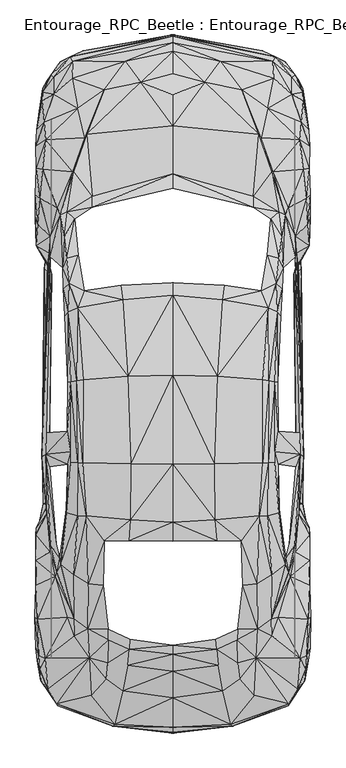
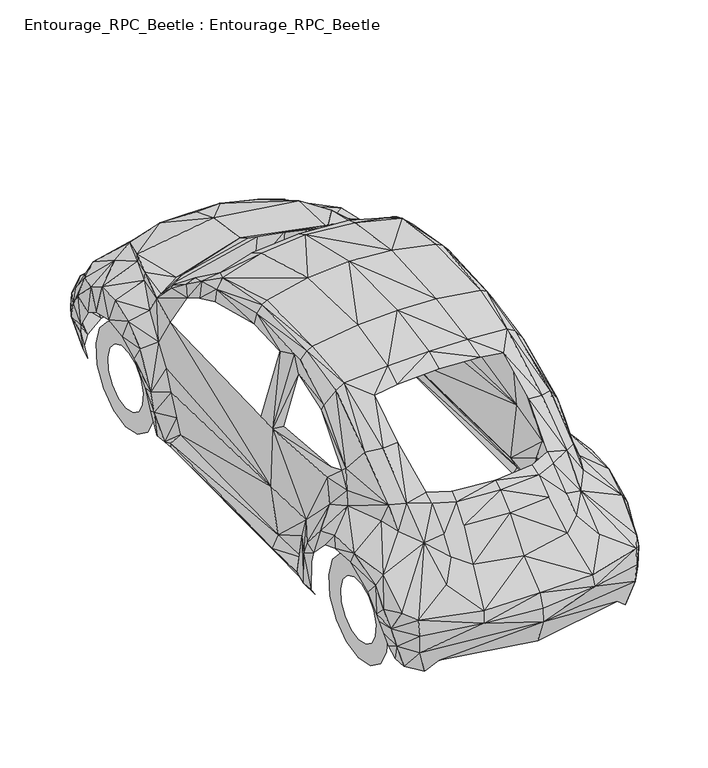
"""IFC4 building model written with IfcOpenShell, lengths in millimetres: proxy geometry, Entourage_RPC_Beetle : Entourage_RPC_Beetle."""

from ifc_helpers import new_model, si_unit, origin, place, context, project, spatial, triangles, source, transform, mapped, element, save


def entourage_rpc_beetle_entourage_rpc_beetle_b6d71803(model_context):
    return source(origin(), model_context, "Body", "Tessellation", [
        triangles([(0.0, -749.071574, 521.742899), (0.0, -720.6335569, 604.033443), (0.0, -697.1470545, 283.3282728), (0.0, -553.0728908, 738.9057701), (0.0, -753.760096, 438.7513078), (0.0, -253.8386484, 1040.4185434), (0.0, -401.3744104, 922.0218458), (0.0, -305.0182643, 1012.9445663), (0.0, 339.5469707, 1396.6602436), (0.0, 448.9171117, 1443.1075539), (0.0, 778.6050184, 1505.0664173), (0.0, 1285.8879353, 1510.4998066), (0.0, 1742.2541199, 1403.2768456), (0.0, 2432.6093651, 967.8556761), (0.0, 3132.1224815, 632.4714237), (0.0, 3003.4724854, 772.0323092), (0.0, 2706.0784286, 929.3833151), (0.0, 3166.3445206, 220.3177475), (0.0, 2885.1195351, 859.3180424), (0.0, 3224.7104347, 396.0724085), (0.0, 3181.1549538, 556.1401817), (0.0, 3216.1220055, 530.6379956), (-338.407687, -715.988855, 523.3642027), (-331.2653541, -702.6243364, 593.8676027), (-244.8997318, -218.1706584, 1034.7659815), (-249.1500901, -276.1420835, 1003.6112698), (-257.9137267, -368.4231514, 912.4695219), (-249.2377301, 343.0524253, 1381.9373051), (-285.431542, -511.8838351, 760.9462852), (-240.2988317, 460.3974792, 1427.552108), (-236.6180971, 781.4093531, 1494.4185207), (-652.9344915, -590.6250681, 370.7455024), (-540.4532759, -593.7361791, 283.6349946), (-181.3633847, 2956.2803078, 806.8677555), (-253.3566466, 1279.4466133, 1497.179108), (-380.1225826, -444.6667534, 798.8051662), (-371.1837024, -353.5687892, 889.7717068), (-368.2478714, -222.3771967, 1004.1371098), (-368.6422514, -160.8126769, 1037.3951088), (-390.4198829, 343.0962453, 1359.9406826), (-282.758631, 1714.4296555, 1400.2533382), (-397.6060358, 87.5486986, 1216.1732225), (-463.4209502, -538.1309249, 705.2972111), (-271.6726434, 3074.4140854, 663.1441154), (-476.0843851, -323.2904411, 850.4230185), (-464.0343939, 3087.9975586, 214.4022838), (-482.5694544, 95.8303334, 1204.2108713), (-485.3738254, -159.4104914, 1005.7583771), (-569.1103566, 3073.5815781, 547.1136251), (-493.874542, 483.577278, 1392.2346416), (-583.6579788, 3101.4935371, 522.400199), (-510.6130915, 3134.4011215, 369.6500387), (-392.1287902, 2913.6012268, 783.2935404), (-656.7905062, -598.249421, 480.4223834), (-660.6903408, -585.2354261, 576.6470695), (-562.669071, -200.2052034, 880.3069502), (-560.43436, -101.5266881, 987.8367239), (-512.8040188, 786.711355, 1449.4173431), (-542.1621832, 485.1109417, 1360.7731899), (-564.3779783, 148.6750366, 1173.0999796), (-608.8972449, -561.6174273, 218.6088402), (-511.6209151, 1259.3779255, 1457.1731197), (-542.7756269, 785.2215477, 1431.62715), (-459.1705556, 2305.6242382, 949.6711029), (-601.448172, -92.8068806, 893.8030014), (-504.0842022, 1766.485635, 1321.8626289), (-546.4125415, 1253.8568962, 1442.4940739), (-603.419963, 501.4989312, 1279.4466133), (-580.5469042, 789.4281223, 1379.6588104), (-607.6265376, 520.2092717, 1235.979063), (-601.6672357, 965.9276688, 1337.9439148), (-712.9654203, -503.4269022, 590.8879881), (-543.0385468, 1671.1811325, 1362.0876446), (-490.9387473, 2659.6751564, 894.1096687), (-600.0459683, 778.6050184, 1308.1913704), (-598.468521, 1244.567347, 1344.6919041), (-640.008173, 208.2677382, 1063.2039986), (-680.8904886, -470.5194632, 218.8279221), (-538.8320086, 1968.0492039, 1181.3815962), (-581.3794478, 1249.0807343, 1402.7071129), (-644.9596149, 243.4537263, 1028.9820322), (-502.6819985, 2637.5907486, 866.5918716), (-661.1722881, 162.3463042, 955.8933249), (-690.7057325, -396.8611321, 226.9780968), (-559.5141764, 2176.4921494, 1011.849139), (-670.6370447, 140.9630437, 873.2960409), (-662.9250154, 324.5173285, 1010.1402317), (-615.5138105, 1624.5585423, 1262.9710201), (-595.0507064, 1647.2125374, 1322.1692963), (-589.8363444, 1810.8295853, 1270.2885967), (-729.3095535, -482.3065707, 373.4622334), (-752.0950087, -454.7449536, 476.8731088), (-694.5179272, 315.5346282, 958.4347395), (-727.0748789, -327.5407994, 736.0575428), (-623.3572271, 1778.4479862, 1193.6068674), (-565.0352783, 2447.3761963, 934.772957), (-732.2892408, -394.1444012, 324.3420848), (-571.3888876, 2445.9300636, 884.7764448), (-699.1188818, 280.0419, 808.1822828), (-604.6907066, 1951.091518, 1171.2596123), (-587.8206971, 3015.1281693, 200.2490234), (-691.4068525, 574.6314222, 283.8102746), (-750.7366613, -381.2618663, 397.2555121), (-627.9581818, 1897.5456585, 1125.469602), (-602.8941593, 2217.067725, 949.8025629), (-619.8517725, 2074.2206303, 1075.9989298), (-710.949773, 550.0056361, 448.9171117), (-765.2404999, -360.5796985, 467.8465522), (-699.9952091, 763.1372126, 1016.187101), (-763.8382599, -313.4313409, 671.3819847), (-758.3609779, -391.2086065, 565.0352783), (-717.9606823, 496.6350929, 583.9647188), (-723.2188643, 461.5367629, 181.1004829), (-718.1359623, 554.8256181, 180.0050374), (-771.9884892, -342.0446016, 511.3579951), (-574.3247186, 2977.4883156, 683.0814159), (-731.2813808, 376.1351443, 185.3070212), (-541.5487395, 2807.2984131, 783.4688204), (-640.183453, 2199.9349045, 944.8949409), (-739.4315374, 551.9336434, 222.5524767), (-782.1104731, -268.9559124, 609.6421486), (-772.8209965, -106.1275973, 756.4330433), (-722.2110043, 958.3909195, 967.6803961), (-703.8074038, 810.6798775, 292.5300731), (-725.3221516, 835.6124399, 965.0075214), (-758.2734106, 370.7893224, 225.6197495), (-785.8788477, -90.0025187, 695.9639145), (-780.1824657, 80.9759712, 676.0266867), (-779.9195457, 89.5643369, 755.1622633), (-760.9024652, 444.4038334, 223.2973804), (-778.6050184, 192.2302905, 631.3321764), (-659.0690735, 2238.6701855, 850.3353785), (-771.4626492, 345.7253363, 426.4822165), (-774.7051838, 315.3593482, 502.0247349), (-781.7160931, 232.4115588, 696.3582945), (-719.7134096, 810.6360575, 185.964303), (-690.3552452, 1860.1249775, 294.1075386), (-697.1470545, 1960.2056419, 957.0763922), (-780.2701057, 377.6249516, 532.7412829), (-778.6488384, 417.2804163, 440.0220151), (-746.0043194, 820.1446341, 614.0678232), (-678.173794, 2886.7845497, 671.0752447), (-698.0233818, 2078.8215122, 757.3970106), (-640.051993, 3071.2590454, 391.9535102), (-713.4911877, 1919.5424263, 537.0792812), (-718.6617296, 1911.1731697, 193.1066541), (-705.6477711, 1983.2978371, 648.7279896), (-731.2813808, 1892.3751892, 233.5070043), (-674.4492393, 2909.8331429, 198.8030179), (-727.3815462, 2040.3052586, 190.0832013), (-722.1233643, 1974.7095531, 190.0832013), (-678.6557413, 2984.5867195, 540.8914395), (-700.0828491, 2817.5957497, 206.339749), (-696.8403145, 2993.6132034, 517.7554607), (-724.1390116, 2626.4609047, 788.1135223), (-699.5570091, 1883.7430126, 390.6389465), (-765.4157072, 2043.5477932, 362.8144094), (-742.2797647, 2459.3385475, 809.2338902), (-716.646155, 2967.1470863, 449.8372953), (-766.9494072, 2002.4902702, 376.836228), (-732.0701408, 2726.2786491, 728.1264862), (-771.6817492, 2086.0077015, 482.5694544), (-759.6317579, 2292.9609123, 780.6206657), (-769.5346418, 2144.7677776, 699.5131891), (-778.0791784, 2024.2239727, 495.1452856), (-742.9808121, 2848.7944267, 602.2807157), (-782.6363131, 2187.1400459, 616.8721579), (-740.0450174, 2920.3932541, 427.6653202), (-741.6224648, 2898.4841263, 520.1654517), (-750.9119413, 2806.3345184, 398.3509395), (-782.7677004, 2314.7385075, 681.1972286), (-778.6050184, 2464.4652695, 693.9921598), (-760.4204453, 2788.5004326, 455.5336773), (-774.7051838, 2684.6515388, 603.0694393), (-780.8835857, 2591.1871857, 666.7810301), (-743.1122721, 809.6720901, 220.5368294), (0.0, 2350.6693085, 1011.849139), (-459.1705556, 2241.4745201, 1007.2920044), (0.0, 1813.2396126, 1369.1424465), (-294.1513586, 1797.0267941, 1360.0720699), (-580.6345442, 850.2915585, 1382.7260651), (338.407687, -715.988855, 523.3642027), (331.2653541, -702.6243364, 593.8676027), (244.8997318, -218.1706584, 1034.7659815), (249.1500901, -276.1420835, 1003.6112698), (257.9137267, -368.4231514, 912.4695219), (249.2377301, 343.0524253, 1381.9373051), (285.431542, -511.8838351, 760.9462852), (240.2988317, 460.3974792, 1427.552108), (236.6180971, 781.4093531, 1494.4185207), (652.9344915, -590.6250681, 370.7455024), (540.4532759, -593.7361791, 283.6349946), (181.3633847, 2956.2803078, 806.8677555), (253.3566466, 1279.4466133, 1497.179108), (380.1225826, -444.6667534, 798.8051662), (371.1837024, -353.5687892, 889.7717068), (368.2478714, -222.3771967, 1004.1371098), (368.6422514, -160.8126769, 1037.3951088), (390.4198829, 343.0962453, 1359.9406826), (282.758631, 1714.4296555, 1400.2533382), (397.6060358, 87.5486986, 1216.1732225), (463.4209502, -538.1309249, 705.2972111), (271.6726434, 3074.4140854, 663.1441154), (476.0843851, -323.2904411, 850.4230185), (464.0343939, 3087.9975586, 214.4022838), (482.5694544, 95.8303334, 1204.2108713), (485.3738254, -159.4104914, 1005.7583771), (569.1103566, 3073.5815781, 547.1136251), (493.874542, 483.577278, 1392.2346416), (583.6579788, 3101.4935371, 522.400199), (510.6130915, 3134.4011215, 369.6500387), (392.1287902, 2913.6012268, 783.2935404), (656.7905062, -598.249421, 480.4223834), (660.6903408, -585.2354261, 576.6470695), (562.669071, -200.2052034, 880.3069502), (560.43436, -101.5266881, 987.8367239), (512.8040188, 786.711355, 1449.4173431), (542.1621832, 485.1109417, 1360.7731899), (564.3779783, 148.6750366, 1173.0999796), (608.8972449, -561.6174273, 218.6088402), (511.6209151, 1259.3779255, 1457.1731197), (542.7756269, 785.2215477, 1431.62715), (459.1705556, 2305.6242382, 949.6711029), (601.448172, -92.8068806, 893.8030014), (504.0842022, 1766.485635, 1321.8626289), (546.4125415, 1253.8568962, 1442.4940739), (603.419963, 501.4989312, 1279.4466133), (580.5469042, 789.4281223, 1379.6588104), (607.6265376, 520.2092717, 1235.979063), (601.6672357, 965.9276688, 1337.9439148), (712.9654203, -503.4269022, 590.8879881), (543.0385468, 1671.1811325, 1362.0876446), (490.9387473, 2659.6751564, 894.1096687), (600.0459683, 778.6050184, 1308.1913704), (598.468521, 1244.567347, 1344.6919041), (640.008173, 208.2677382, 1063.2039986), (680.9343086, -470.5194632, 218.8279221), (538.8320086, 1968.0492039, 1181.3815962), (581.3794478, 1249.0807343, 1402.7071129), (644.9596149, 243.4537263, 1028.9820322), (502.6819985, 2637.5907486, 866.5918716), (661.1722881, 162.3463042, 955.8933249), (690.7057325, -396.8611321, 226.9780968), (559.5141764, 2176.4921494, 1011.849139), (670.6370447, 140.9630437, 873.2960409), (662.9250154, 324.5173285, 1010.1402317), (615.5138105, 1624.5585423, 1262.9710201), (595.0507064, 1647.2125374, 1322.1692963), (589.8363444, 1810.8295853, 1270.2885967), (729.3095535, -482.3065707, 373.4622334), (752.0950087, -454.7449536, 476.8731088), (694.5179272, 315.5346282, 958.4347395), (727.0748789, -327.5407994, 736.0575428), (623.3572271, 1778.4479862, 1193.6068674), (565.0352783, 2447.3761963, 934.772957), (732.2892408, -394.1444012, 324.3420848), (571.3888876, 2445.9300636, 884.7764448), (699.1188818, 280.0419, 808.1822828), (604.6907066, 1951.091518, 1171.2596123), (587.8206971, 3015.1281693, 200.2490234), (691.4068525, 574.6314222, 283.8102746), (750.7366613, -381.2618663, 397.2555121), (627.9581818, 1897.5456585, 1125.469602), (602.8941593, 2217.067725, 949.8025629), (619.8517725, 2074.2206303, 1075.9989298), (710.949773, 550.0056361, 448.9171117), (765.2404999, -360.5796985, 467.8465522), (699.9952091, 763.1372126, 1016.187101), (763.8382599, -313.4313409, 671.3819847), (758.3609779, -391.2086065, 565.0352783), (717.9606823, 496.6350929, 583.9647188), (723.2188643, 461.5367629, 181.1004829), (718.1359623, 554.8256181, 180.0050374), (771.9884892, -342.0446016, 511.3579951), (574.3247186, 2977.4883156, 683.0814159), (731.2813808, 376.1351443, 185.3070212), (541.5487395, 2807.2984131, 783.4688204), (640.183453, 2199.9349045, 944.8949409), (739.4315374, 551.9336434, 222.5524767), (782.1104731, -268.9559124, 609.6421486), (772.8209965, -106.1275973, 756.4330433), (722.2548243, 958.3909195, 967.6803961), (703.8074038, 810.6798775, 292.5300731), (725.3221516, 835.6124399, 965.0075214), (758.2734106, 370.7893224, 225.6197495), (785.8788477, -90.0025187, 695.9639145), (780.1824657, 80.9759712, 676.0266867), (779.9633657, 89.5643369, 755.1622633), (760.9024652, 444.4038334, 223.2973804), (778.6050184, 192.2302905, 631.3321764), (659.0690735, 2238.6701855, 850.3353785), (771.4626492, 345.7253363, 426.4822165), (774.7051838, 315.3593482, 502.0247349), (781.7160931, 232.4115588, 696.3582945), (719.7134096, 810.6360575, 185.964303), (690.3552452, 1860.1249775, 294.1075386), (697.1470545, 1960.2056419, 957.0763922), (780.2701057, 377.6249516, 532.7412829), (778.6488384, 417.2804163, 440.0220151), (746.0043194, 820.1446341, 614.0678232), (678.173794, 2886.7845497, 671.0752447), (698.0233818, 2078.8215122, 757.3970106), (640.051993, 3071.2590454, 391.9535102), (713.4911877, 1919.5424263, 537.0792812), (718.6617296, 1911.1731697, 193.1066541), (705.6477711, 1983.2978371, 648.7279896), (731.2813808, 1892.3751892, 233.5070043), (674.4492393, 2909.8331429, 198.8030179), (727.3815462, 2040.3052586, 190.0832013), (722.1233643, 1974.7095531, 190.0832013), (678.6557413, 2984.5867195, 540.8914395), (700.0828491, 2817.5957497, 206.339749), (696.8403145, 2993.6132034, 517.7554607), (724.1390116, 2626.4609047, 788.1135223), (699.5570091, 1883.7430126, 390.6389465), (765.4157072, 2043.5477932, 362.8144094), (742.2797647, 2459.3385475, 809.2338902), (716.646155, 2967.1470863, 449.8372953), (766.9494072, 2002.4902702, 376.836228), (732.0701408, 2726.2786491, 728.1264862), (771.7255692, 2086.0077015, 482.5694544), (759.6317579, 2292.9609123, 780.6206657), (769.5346418, 2144.7677776, 699.5131891), (778.0791784, 2024.2239727, 495.1452856), (742.9808121, 2848.7944267, 602.2807157), (782.6363131, 2187.1400459, 616.8721579), (740.0450174, 2920.3932541, 427.6653202), (741.6224648, 2898.4841263, 520.1654517), (750.9119413, 2806.3345184, 398.3509395), (782.7677004, 2314.7385075, 681.1972286), (778.6050184, 2464.4652695, 693.9921598), (760.4204453, 2788.5004326, 455.5336773), (774.7051838, 2684.6515388, 603.0694393), (780.8835857, 2591.1871857, 666.7810301), (743.1122721, 809.6720901, 220.5368294), (459.1705556, 2241.4745201, 1007.2920044), (294.1513586, 1797.0267941, 1360.0720699), (580.6345442, 850.2915585, 1382.7260651), (-693.6415998, 2431.9082451, 0.0015117), (-693.6415998, 2431.9082451, 117.9161946), (-693.6415998, 2558.8496246, 26.9935036), (-693.6415998, 2509.4663017, 134.3918332), (-693.6415998, 2663.794091, 103.2371124), (-693.6415998, 2573.6600578, 181.0143508), (-693.6415998, 2728.6886765, 215.6307153), (-693.6415998, 2613.3154861, 249.7212399), (-693.6415998, 2742.2724403, 344.6752187), (-693.6415998, 2621.5972481, 328.5939328), (-693.6415998, 2702.1786667, 468.1109982), (-693.6415998, 2597.102813, 404.0050275), (-693.6415998, 2615.3310608, 564.5109644), (-693.6415998, 2544.0389008, 462.9404563), (-693.6415998, 2496.8028305, 617.3118113), (-693.6415998, 2471.5636734, 495.2344517), (-693.6415998, 2367.0135143, 617.3118113), (-693.6415998, 2392.2528168, 495.2344517), (-693.6415998, 2248.4854294, 564.5109644), (-693.6415998, 2319.7775894, 462.9404563), (-693.6415998, 2161.6378235, 468.1109982), (-693.6415998, 2266.7138226, 404.0050275), (-693.6415998, 2121.5441952, 344.6752187), (-693.6415998, 2242.2193874, 328.5939328), (-693.6415998, 2135.1278137, 215.6307153), (-693.6415998, 2250.501004, 249.7212399), (-693.6415998, 2200.0225445, 103.2371124), (-693.6415998, 2290.1564323, 181.0143508), (-693.6415998, 2304.9670109, 26.9935036), (-693.6415998, 2354.3500431, 134.3918332), (693.6415998, 2431.9082451, 0.0015117), (693.6415998, 2431.9082451, 117.9161946), (693.6415998, 2304.9670109, 26.9935036), (693.6415998, 2354.3500431, 134.3918332), (693.6415998, 2200.0225445, 103.2371124), (693.6415998, 2290.1564323, 181.0143508), (693.6415998, 2135.1278137, 215.6307153), (693.6415998, 2250.501004, 249.7212399), (693.6415998, 2121.5441952, 344.6752187), (693.6415998, 2242.2193874, 328.5939328), (693.6415998, 2161.6378235, 468.1109982), (693.6415998, 2266.7138226, 404.0050275), (693.6415998, 2248.4854294, 564.5109644), (693.6415998, 2319.7775894, 462.9404563), (693.6415998, 2367.0135143, 617.3118113), (693.6415998, 2392.2528168, 495.2344517), (693.6415998, 2496.8028305, 617.3118113), (693.6415998, 2471.5636734, 495.2344517), (693.6415998, 2615.3310608, 564.5109644), (693.6415998, 2544.0389008, 462.9404563), (693.6415998, 2702.1786667, 468.1109982), (693.6415998, 2597.102813, 404.0050275), (693.6415998, 2742.2724403, 344.6752187), (693.6415998, 2621.5972481, 328.5939328), (693.6415998, 2728.6886765, 215.6307153), (693.6415998, 2613.3154861, 249.7212399), (693.6415998, 2663.794091, 103.2371124), (693.6415998, 2573.6600578, 181.0143508), (693.6415998, 2558.8496246, 26.9935036), (693.6415998, 2509.4663017, 134.3918332), (-693.6415998, -13.5836322, 0.0015117), (-693.6415998, -13.5836322, 117.9161946), (-693.6415998, 113.3575975, 26.9935036), (-693.6415998, 63.9745244, 134.3918332), (-693.6415998, 218.3021002, 103.2371124), (-693.6415998, 128.1681397, 181.0143508), (-693.6415998, 283.1968128, 215.6307153), (-693.6415998, 167.8235862, 249.7212399), (-693.6415998, 296.7804495, 344.6752187), (-693.6415998, 176.1052209, 328.5939328), (-693.6415998, 256.6868212, 468.1109982), (-693.6415998, 151.6108585, 404.0050275), (-693.6415998, 169.8392153, 564.5109644), (-693.6415998, 98.5470553, 462.9404563), (-693.6415998, 51.3110713, 617.3118113), (-693.6415998, 26.0718098, 495.2344517), (-693.6415998, -78.4783402, 617.3118113), (-693.6415998, -53.2390741, 495.2344517), (-693.6415998, -197.0064706, 564.5109644), (-693.6415998, -125.7143196, 462.9404563), (-693.6415998, -283.8540765, 468.1109982), (-693.6415998, -178.7781137, 404.0050275), (-693.6415998, -323.9477048, 344.6752187), (-693.6415998, -203.2724762, 328.5939328), (-693.6415998, -310.3640862, 215.6307153), (-693.6415998, -194.9908414, 249.7212399), (-693.6415998, -245.4693737, 103.2371124), (-693.6415998, -155.335395, 181.0143508), (-693.6415998, -140.5248618, 26.9935036), (-693.6415998, -91.1417842, 134.3918332), (693.6415998, -13.5836322, 0.0015117), (693.6415998, -13.5836322, 117.9161946), (693.6415998, -140.5248618, 26.9935036), (693.6415998, -91.1417842, 134.3918332), (693.6415998, -245.4693737, 103.2371124), (693.6415998, -155.335395, 181.0143508), (693.6415998, -310.3640862, 215.6307153), (693.6415998, -194.9908414, 249.7212399), (693.6415998, -323.9477048, 344.6752187), (693.6415998, -203.2724762, 328.5939328), (693.6415998, -283.8540765, 468.1109982), (693.6415998, -178.7781137, 404.0050275), (693.6415998, -197.0064706, 564.5109644), (693.6415998, -125.7143196, 462.9404563), (693.6415998, -78.4783402, 617.3118113), (693.6415998, -53.2390741, 495.2344517), (693.6415998, 51.3110713, 617.3118113), (693.6415998, 26.0718098, 495.2344517), (693.6415998, 169.8392153, 564.5109644), (693.6415998, 98.5470553, 462.9404563), (693.6415998, 256.6868212, 468.1109982), (693.6415998, 151.6108585, 404.0050275), (693.6415998, 296.7804495, 344.6752187), (693.6415998, 176.1052209, 328.5939328), (693.6415998, 283.1968128, 215.6307153), (693.6415998, 167.8235862, 249.7212399), (693.6415998, 218.3021002, 103.2371124), (693.6415998, 128.1681397, 181.0143508), (693.6415998, 113.3575975, 26.9935036), (693.6415998, 63.9745244, 134.3918332)], [[67, 58, 62], [67, 63, 58], [53, 82, 74], [34, 17, 19], [118, 82, 53], [155, 98, 82], [155, 158, 98], [34, 74, 17], [172, 155, 175], [172, 158, 155], [159, 168, 169], [166, 142, 169], [175, 161, 174], [175, 155, 161], [142, 152, 169], [154, 169, 152], [160, 145, 165], [160, 156, 145], [162, 160, 165], [162, 157, 160], [34, 53, 74], [74, 96, 64], [82, 96, 74], [82, 98, 96], [36, 29, 27], [29, 43, 24], [23, 55, 54], [23, 24, 55], [23, 2, 24], [23, 1, 2], [5, 1, 23], [134, 140, 133], [134, 139, 140], [117, 130, 113], [117, 126, 130], [113, 120, 114], [113, 130, 120], [140, 112, 107], [140, 139, 112], [92, 108, 103], [91, 103, 97], [91, 92, 103], [61, 33, 32], [84, 78, 91], [84, 91, 97], [38, 26, 25], [77, 81, 83], [63, 50, 58], [63, 59, 50], [68, 63, 69], [68, 59, 63], [181, 75, 69], [74, 64, 17], [64, 14, 17], [64, 178, 14], [178, 177, 14], [34, 19, 16], [53, 34, 44], [21, 44, 15], [21, 49, 44], [44, 34, 15], [34, 16, 15], [22, 49, 21], [22, 51, 49], [20, 51, 22], [20, 52, 51], [18, 52, 20], [18, 46, 52], [51, 152, 49], [51, 154, 152], [101, 144, 46], [144, 52, 46], [101, 159, 144], [159, 169, 154], [101, 168, 159], [101, 149, 168], [149, 170, 168], [149, 153, 170], [168, 173, 169], [168, 170, 173], [49, 142, 116], [49, 152, 142], [49, 116, 44], [116, 142, 118], [161, 155, 118], [155, 82, 118], [142, 161, 118], [158, 132, 98], [158, 163, 132], [172, 163, 158], [172, 171, 163], [98, 119, 96], [98, 132, 119], [171, 164, 163], [171, 167, 164], [163, 143, 132], [163, 164, 143], [96, 105, 64], [96, 119, 105], [105, 178, 64], [105, 85, 178], [167, 165, 164], [167, 162, 165], [165, 143, 164], [165, 147, 143], [150, 160, 157], [150, 151, 160], [151, 156, 160], [151, 148, 137], [13, 35, 12], [13, 41, 35], [12, 31, 11], [12, 35, 31], [35, 58, 31], [35, 62, 58], [11, 30, 10], [11, 31, 30], [31, 50, 30], [31, 58, 50], [10, 28, 9], [10, 30, 28], [30, 40, 28], [30, 50, 40], [125, 75, 181], [125, 109, 75], [125, 87, 109], [125, 93, 87], [123, 141, 125], [137, 141, 156], [137, 124, 141], [148, 124, 137], [148, 176, 124], [146, 176, 148], [146, 136, 176], [141, 112, 125], [112, 93, 125], [112, 99, 93], [124, 112, 141], [124, 107, 112], [124, 102, 107], [176, 102, 124], [176, 120, 102], [136, 120, 176], [136, 114, 120], [47, 40, 50], [47, 42, 40], [48, 42, 47], [48, 39, 42], [57, 47, 60], [57, 48, 47], [60, 50, 59], [60, 47, 50], [59, 77, 60], [59, 68, 77], [77, 57, 60], [77, 83, 57], [70, 77, 68], [70, 81, 77], [75, 68, 69], [75, 70, 68], [26, 6, 25], [26, 8, 6], [27, 8, 26], [27, 7, 8], [29, 7, 27], [29, 4, 7], [24, 4, 29], [24, 2, 4], [32, 5, 23], [33, 5, 32], [33, 3, 5], [32, 23, 54], [55, 45, 72], [55, 24, 43], [99, 83, 93], [99, 86, 83], [135, 86, 99], [135, 129, 86], [131, 129, 135], [131, 128, 129], [93, 81, 87], [93, 83, 81], [128, 122, 129], [128, 127, 122], [122, 86, 129], [122, 65, 86], [86, 57, 83], [86, 65, 57], [127, 110, 122], [127, 121, 110], [110, 94, 122], [122, 94, 65], [94, 56, 65], [56, 57, 65], [56, 48, 57], [56, 45, 48], [94, 45, 56], [115, 110, 121], [115, 111, 110], [111, 94, 110], [111, 72, 94], [108, 92, 115], [92, 111, 115], [78, 32, 91], [78, 61, 32], [45, 38, 48], [45, 37, 38], [37, 26, 38], [37, 27, 26], [36, 27, 37], [134, 135, 139], [134, 131, 135], [139, 99, 112], [139, 135, 99], [126, 140, 130], [126, 133, 140], [130, 107, 120], [130, 140, 107], [120, 107, 102], [45, 36, 37], [92, 55, 72], [92, 54, 55], [91, 54, 92], [91, 32, 54], [92, 72, 111], [72, 45, 94], [43, 45, 55], [43, 36, 45], [43, 29, 36], [79, 90, 66], [79, 100, 90], [90, 73, 66], [85, 100, 79], [85, 106, 100], [85, 105, 106], [105, 119, 106], [95, 88, 89], [90, 89, 73], [89, 67, 73], [73, 67, 62], [89, 76, 80], [89, 80, 67], [88, 76, 89], [73, 35, 41], [73, 62, 35], [69, 63, 181], [80, 63, 67], [76, 71, 80], [146, 148, 151], [141, 147, 145], [151, 137, 156], [173, 166, 169], [173, 174, 166], [166, 174, 161], [166, 161, 142], [52, 144, 51], [144, 154, 51], [144, 159, 154], [116, 53, 44], [116, 118, 53], [119, 143, 138], [143, 119, 132], [143, 147, 138], [138, 104, 119], [119, 104, 106], [104, 100, 106], [104, 90, 100], [104, 95, 90], [95, 89, 90], [25, 39, 38], [38, 39, 48], [141, 138, 147], [156, 141, 145], [165, 145, 147], [41, 179, 180], [41, 13, 179], [66, 41, 180], [66, 73, 41], [123, 125, 71], [125, 181, 71], [71, 181, 80], [181, 63, 80], [138, 141, 123], [226, 221, 217], [226, 217, 222], [212, 233, 241], [193, 19, 17], [277, 212, 241], [314, 241, 257], [314, 257, 317], [193, 17, 233], [331, 334, 314], [331, 314, 317], [318, 328, 327], [325, 328, 301], [334, 333, 320], [334, 320, 314], [301, 328, 311], [313, 311, 328], [319, 324, 304], [319, 304, 315], [321, 324, 319], [321, 319, 316], [193, 233, 212], [233, 223, 255], [241, 233, 255], [241, 255, 257], [195, 186, 188], [188, 183, 202], [182, 213, 214], [182, 214, 183], [182, 183, 2], [182, 2, 1], [5, 182, 1], [293, 292, 299], [293, 299, 298], [276, 272, 289], [276, 289, 285], [272, 273, 279], [272, 279, 289], [299, 266, 271], [299, 271, 298], [251, 262, 267], [250, 256, 262], [250, 262, 251], [220, 191, 192], [243, 250, 237], [243, 256, 250], [197, 184, 185], [236, 242, 240], [222, 217, 209], [222, 209, 218], [227, 228, 222], [227, 222, 218], [338, 228, 234], [233, 17, 223], [223, 17, 14], [223, 14, 336], [336, 14, 177], [193, 16, 19], [212, 203, 193], [21, 15, 203], [21, 203, 208], [203, 15, 193], [193, 15, 16], [22, 21, 208], [22, 208, 210], [20, 22, 210], [20, 210, 211], [18, 20, 211], [18, 211, 205], [210, 208, 311], [210, 311, 313], [260, 205, 303], [303, 205, 211], [260, 303, 318], [318, 313, 328], [260, 318, 327], [260, 327, 308], [308, 327, 329], [308, 329, 312], [327, 328, 332], [327, 332, 329], [208, 275, 301], [208, 301, 311], [208, 203, 275], [275, 277, 301], [320, 277, 314], [314, 277, 241], [301, 277, 320], [317, 257, 291], [317, 291, 322], [331, 317, 322], [331, 322, 330], [257, 255, 278], [257, 278, 291], [330, 322, 323], [330, 323, 326], [322, 291, 302], [322, 302, 323], [255, 223, 264], [255, 264, 278], [264, 223, 336], [264, 336, 244], [326, 323, 324], [326, 324, 321], [324, 323, 302], [324, 302, 306], [309, 316, 319], [309, 319, 310], [310, 319, 315], [310, 296, 307], [13, 12, 194], [13, 194, 200], [12, 11, 190], [12, 190, 194], [194, 190, 217], [194, 217, 221], [11, 10, 189], [11, 189, 190], [190, 189, 209], [190, 209, 217], [10, 9, 187], [10, 187, 189], [189, 187, 199], [189, 199, 209], [284, 338, 234], [284, 234, 268], [284, 268, 246], [284, 246, 252], [282, 284, 300], [296, 315, 300], [296, 300, 283], [307, 296, 283], [307, 283, 335], [305, 307, 335], [305, 335, 295], [300, 284, 271], [271, 284, 252], [271, 252, 258], [283, 300, 271], [283, 271, 266], [283, 266, 261], [335, 283, 261], [335, 261, 279], [295, 335, 279], [295, 279, 273], [206, 209, 199], [206, 199, 201], [207, 206, 201], [207, 201, 198], [216, 219, 206], [216, 206, 207], [219, 218, 209], [219, 209, 206], [218, 219, 236], [218, 236, 227], [236, 219, 216], [236, 216, 242], [229, 227, 236], [229, 236, 240], [234, 228, 227], [234, 227, 229], [185, 184, 6], [185, 6, 8], [186, 185, 8], [186, 8, 7], [188, 186, 7], [188, 7, 4], [183, 188, 4], [183, 4, 2], [191, 182, 5], [192, 191, 5], [192, 5, 3], [191, 213, 182], [214, 231, 204], [214, 202, 183], [258, 252, 242], [258, 242, 245], [294, 258, 245], [294, 245, 288], [290, 294, 288], [290, 288, 287], [252, 246, 240], [252, 240, 242], [287, 288, 281], [287, 281, 286], [281, 288, 245], [281, 245, 224], [245, 242, 216], [245, 216, 224], [286, 281, 269], [286, 269, 280], [269, 281, 253], [281, 224, 253], [253, 224, 215], [215, 224, 216], [215, 216, 207], [215, 207, 204], [253, 215, 204], [274, 280, 269], [274, 269, 270], [270, 269, 253], [270, 253, 231], [267, 274, 251], [251, 274, 270], [237, 250, 191], [237, 191, 220], [204, 207, 197], [204, 197, 196], [196, 197, 185], [196, 185, 186], [195, 196, 186], [293, 298, 294], [293, 294, 290], [298, 271, 258], [298, 258, 294], [285, 289, 299], [285, 299, 292], [289, 279, 266], [289, 266, 299], [279, 261, 266], [204, 196, 195], [251, 231, 214], [251, 214, 213], [250, 251, 213], [250, 213, 191], [251, 270, 231], [231, 253, 204], [202, 214, 204], [202, 204, 195], [202, 195, 188], [238, 225, 249], [238, 249, 259], [249, 225, 232], [244, 238, 259], [244, 259, 265], [244, 265, 264], [264, 265, 278], [254, 248, 247], [249, 232, 248], [248, 232, 226], [232, 221, 226], [248, 239, 235], [248, 226, 239], [247, 248, 235], [232, 200, 194], [232, 194, 221], [228, 338, 222], [239, 226, 222], [235, 239, 230], [305, 310, 307], [300, 304, 306], [310, 315, 296], [332, 328, 325], [332, 325, 333], [325, 320, 333], [325, 301, 320], [211, 210, 303], [303, 210, 313], [303, 313, 318], [275, 203, 212], [275, 212, 277], [278, 297, 302], [302, 291, 278], [302, 297, 306], [297, 278, 263], [278, 265, 263], [263, 265, 259], [263, 259, 249], [263, 249, 254], [254, 249, 248], [184, 197, 198], [197, 207, 198], [300, 306, 297], [315, 304, 300], [324, 306, 304], [200, 337, 179], [200, 179, 13], [225, 337, 200], [225, 200, 232], [282, 230, 284], [284, 230, 338], [230, 239, 338], [338, 239, 222], [297, 282, 300], [339, 342, 341], [339, 340, 342], [341, 344, 343], [341, 342, 344], [343, 346, 345], [343, 344, 346], [345, 348, 347], [345, 346, 348], [347, 350, 349], [347, 348, 350], [349, 352, 351], [349, 350, 352], [351, 354, 353], [351, 352, 354], [353, 356, 355], [353, 354, 356], [355, 358, 357], [355, 356, 358], [357, 360, 359], [357, 358, 360], [359, 362, 361], [359, 360, 362], [361, 364, 363], [361, 362, 364], [363, 366, 365], [363, 364, 366], [365, 368, 367], [365, 366, 368], [367, 340, 339], [367, 368, 340], [369, 372, 371], [369, 370, 372], [371, 374, 373], [371, 372, 374], [373, 376, 375], [373, 374, 376], [375, 378, 377], [375, 376, 378], [377, 380, 379], [377, 378, 380], [379, 382, 381], [379, 380, 382], [381, 384, 383], [381, 382, 384], [383, 386, 385], [383, 384, 386], [385, 388, 387], [385, 386, 388], [387, 390, 389], [387, 388, 390], [389, 392, 391], [389, 390, 392], [391, 394, 393], [391, 392, 394], [393, 396, 395], [393, 394, 396], [395, 398, 397], [395, 396, 398], [397, 370, 369], [397, 398, 370], [399, 402, 401], [399, 400, 402], [401, 404, 403], [401, 402, 404], [403, 406, 405], [403, 404, 406], [405, 408, 407], [405, 406, 408], [407, 410, 409], [407, 408, 410], [409, 412, 411], [409, 410, 412], [411, 414, 413], [411, 412, 414], [413, 416, 415], [413, 414, 416], [415, 418, 417], [415, 416, 418], [417, 420, 419], [417, 418, 420], [419, 422, 421], [419, 420, 422], [421, 424, 423], [421, 422, 424], [423, 426, 425], [423, 424, 426], [425, 428, 427], [425, 426, 428], [427, 400, 399], [427, 428, 400], [429, 432, 431], [429, 430, 432], [431, 434, 433], [431, 432, 434], [433, 436, 435], [433, 434, 436], [435, 438, 437], [435, 436, 438], [437, 440, 439], [437, 438, 440], [439, 442, 441], [439, 440, 442], [441, 444, 443], [441, 442, 444], [443, 446, 445], [443, 444, 446], [445, 448, 447], [445, 446, 448], [447, 450, 449], [447, 448, 450], [449, 452, 451], [449, 450, 452], [451, 454, 453], [451, 452, 454], [453, 456, 455], [453, 454, 456], [455, 458, 457], [455, 456, 458], [457, 430, 429], [457, 458, 430]], closed=False),
    ])


if __name__ == "__main__":
    model = new_model("IFC4")
    model_context = context("Model", 3, world=origin())
    ifc_project = project(units=[si_unit("LENGTHUNIT", "METRE", prefix="MILLI")], contexts=[model_context])
    site = spatial("IfcSite", under=ifc_project)
    building = spatial("IfcBuilding", under=site)
    placement = place(None, origin())
    entourage_rpc_beetle_entourage_rpc_beetle_shape = entourage_rpc_beetle_entourage_rpc_beetle_b6d71803(model_context)
    element("IfcBuildingElementProxy", 1, Name="Entourage_RPC_Beetle : Entourage_RPC_Beetle", ObjectType="Entourage_RPC_Beetle : Entourage_RPC_Beetle", at=placement, inside=building, context=model_context, shape_type="MappedRepresentation", body=[
        mapped(entourage_rpc_beetle_entourage_rpc_beetle_shape, transform((0.0, 0.0, 0.0), x_axis=(1.0, 0.0, 0.0), y_axis=(0.0, 1.0, 0.0), z_axis=(0.0, 0.0, 1.0))),
    ])
    save(model, "model.ifc")

# Revit data of these elements
# Type "Entourage_RPC_Beetle : Entourage_RPC_Beetle"
#   built-in parameter 1005198 = "{2, 15},{39, RPC-16-0U6E-L4EG-ENH1-J3KF-SVEL-0TX4-C0},{1, 0},{1, 0},{2, 18},{1, 8},{5, Color},{1, 0},{1, 0},{3, 0.8},{3, 0.8},{3, 0.8},{1, 8},{7, BBoxMin},{1, 0},{1, 0},{1, 0},{1, 0},{1, 0},{1, 8},{7, BBoxMax},{1, 0},{1, 0},{1, 0},{1, 0},{1, 0},{2, 11},{9, RPCTypeId},{1, 0},{1, 0},{39, RPC-16-0U6E-L4EG-ENH1-J3KF-SVEL-0TX4-C0},{1, 6},{14, RPCPlantHeight},{1, 0},{1, 0},{4, 4.92},{2, 11},{7, keyword},{1, 0},{1, 0},{39, :RPCs:Auto_Economy/Midsize:Geometry:RPC},{2, 11},{8, category},{1, 0},{1, 0},{20, Auto_Economy/Midsize},{2, 11},{12, LocalizedUID},{1, 0},{1, 0},{13, VW Beetle [4]},{2, 14},{6, Height},{1, 0},{1, 0},{4, 4.92},{1, 2},{16, Cast Reflections},{1, 0},{1, 0},{1, 0},{1, 4},{12, Transparency},{1, 0},{1, 0},{2, 18},{1, 4},{7, Tinting},{1, 0},{1, 0},{2, 50},{1, 2},{11, Use Tinting},{1, 0},{1, 0},{1, 0},{1, 2},{13, License Plate},{1, 0},{1, 0},{1, 0},{2, 11},{21, License Plate Texture},{1, 0},{1, 0},{64, __RPC:/object data/textures/car/plate/textures/default/rgb/0/0/0},{2, 11},{23, i_License Plate Texture},{1, 0},{1, 0},{0, },{1, 2},{12, Custom Plate},{1, 0},{1, 0},{1, 0},{2, 11},{23, License Plate File Name},{1, 0},{1, 0},{0, },{21, assetlibrary_base.fbx},{1, 5},"
#   built-in parameter 1005195 = "RPC-16-0U6E-L4EG-ENH1-J3KF-SVEL-0TX4-C0"
#   Height = 0
